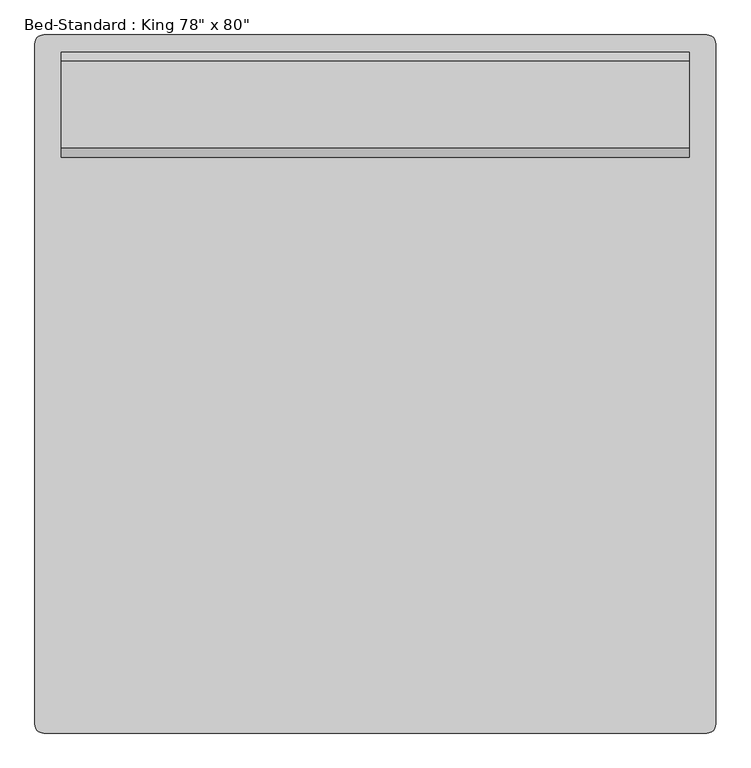
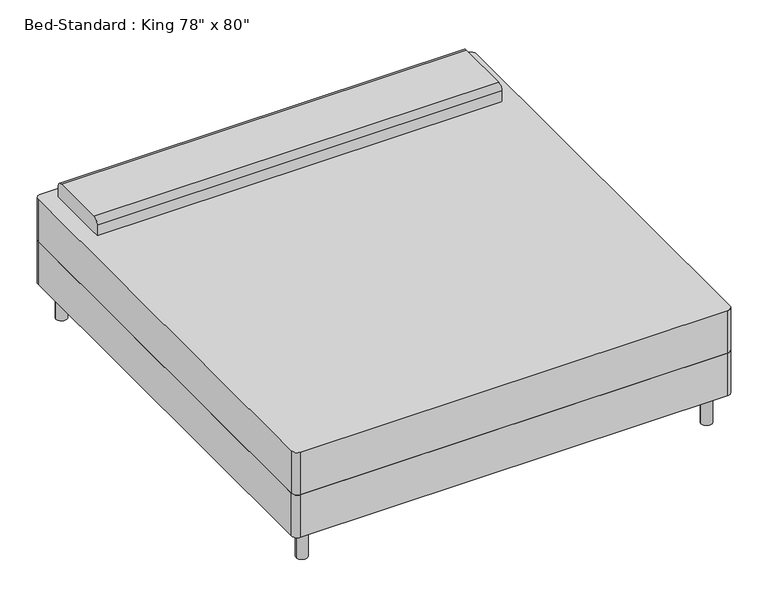
"""IFC4 building model written with IfcOpenShell, lengths in millimetres: furniture geometry."""

import ifcopenshell
import ifcopenshell.guid

model = None  # the IFC model being written
_history = None  # IfcOwnerHistory: only IFC2X3 demands one
_inside = {}  # id of a spatial element -> (the spatial element, [elements in it])
_under = {}  # id of a project, library or spatial element -> (it, [spatial elements below it])
_declared = {}  # id of a project -> (the project, [libraries it declares])
_typed = {}  # id of a type object -> (the type object, [elements of that type])
_made_of = {}  # id of a material, layer set ... -> (it, [elements and type objects made of it])


def new_model(schema):
    """Start an empty IFC model of exactly this schema.

    Asked for "IFC4X3", IfcOpenShell would pick the latest addendum, in which some entities
    have other attributes; the version numbers below select the first issue.
    IFC2X3 requires an IfcOwnerHistory on every rooted entity: one is made here for all.
    """
    global model, _history
    if schema == "IFC4X3":
        model = ifcopenshell.file(schema_version=(4, 3, 0, 0))
    else:
        model = ifcopenshell.file(schema=schema)
    _inside.clear()
    _under.clear()
    _declared.clear()
    _typed.clear()
    _made_of.clear()
    _history = None
    if model.schema == "IFC2X3":
        org = make("IfcOrganization", Name="unknown")
        user = make(
            "IfcPersonAndOrganization",
            ThePerson=make("IfcPerson", FamilyName="unknown"),
            TheOrganization=org,
        )
        app = make(
            "IfcApplication",
            ApplicationDeveloper=org,
            Version="unknown",
            ApplicationFullName="unknown",
            ApplicationIdentifier="unknown",
        )
        _history = make(
            "IfcOwnerHistory",
            OwningUser=user,
            OwningApplication=app,
            ChangeAction="ADDED",
            CreationDate=0,
        )
    return model


def make(cls, **values):
    """One entity of the class cls with the attributes given. An attribute that is None is left unset."""
    return model.create_entity(
        cls, **{name: value for name, value in values.items() if value is not None}
    )


def rooted(cls, **values):
    """An entity with a GlobalId (a new one), such as an element, a storey or a relation."""
    return make(cls, GlobalId=ifcopenshell.guid.new(), OwnerHistory=_history, **values)


def si_unit(unit_type, name, prefix=None):
    """IfcSIUnit, for example si_unit("LENGTHUNIT", "METRE", prefix="MILLI")."""
    return make("IfcSIUnit", UnitType=unit_type, Prefix=prefix, Name=name)


def assignment(units):
    """IfcUnitAssignment: the units of a project."""
    return None if units is None else make("IfcUnitAssignment", Units=units)


def point(xyz):
    """IfcCartesianPoint."""
    return None if xyz is None else make("IfcCartesianPoint", Coordinates=xyz)


def direction(xyz):
    """IfcDirection."""
    return None if xyz is None else make("IfcDirection", DirectionRatios=xyz)


def frame(location, z_axis=None, x_axis=None):
    """IfcAxis2Placement3D, a coordinate frame: its origin and axes. An axis left out is left unset."""
    return make(
        "IfcAxis2Placement3D",
        Location=point(location),
        Axis=direction(z_axis),
        RefDirection=direction(x_axis),
    )


def frame_2d(location, x_axis=None):
    """IfcAxis2Placement2D, a coordinate frame in the plane: its origin and x axis."""
    return make(
        "IfcAxis2Placement2D", Location=point(location), RefDirection=direction(x_axis)
    )


def origin():
    """The frame at (0, 0, 0) with its axes left unset."""
    return frame((0.0, 0.0, 0.0))


def origin_with_axes():
    """The frame at (0, 0, 0) with the z axis (0, 0, 1) and the x axis (1, 0, 0) written out."""
    return frame((0.0, 0.0, 0.0), z_axis=(0.0, 0.0, 1.0), x_axis=(1.0, 0.0, 0.0))


def place(relative_to, where):
    """IfcLocalPlacement: puts the frame where relative to a parent placement (None: the world)."""
    return make(
        "IfcLocalPlacement", PlacementRelTo=relative_to, RelativePlacement=where
    )


def context(
    kind, dimensions, precision=None, world=None, true_north=None, identifier=None
):
    """IfcGeometricRepresentationContext, for example the 3D "Model" context."""
    return make(
        "IfcGeometricRepresentationContext",
        ContextIdentifier=identifier,
        ContextType=kind,
        CoordinateSpaceDimension=dimensions,
        Precision=precision,
        WorldCoordinateSystem=world,
        TrueNorth=true_north,
    )


def project(units=None, contexts=None):
    """IfcProject with its units and contexts."""
    return rooted(
        "IfcProject",
        Name="project",
        RepresentationContexts=contexts,
        UnitsInContext=assignment(units),
    )


def spatial(cls, under=None, at=None, **own):
    """A site, building, storey or space (cls), placed at a placement, below another one or the project."""
    s = rooted(cls, ObjectPlacement=at, **own)
    if under is not None:
        _under.setdefault(under.id(), (under, []))[1].append(s)
    return s


def polyline(points):
    """IfcPolyline through the points."""
    return make("IfcPolyline", Points=[point(p) for p in points])


def circle_curve(where, radius):
    """IfcCircle in the frame where."""
    return make("IfcCircle", Position=where, Radius=radius)


def trimmed(basis, trim1, trim2, sense, master):
    """IfcTrimmedCurve: the piece of a basis curve between two trims."""
    return make(
        "IfcTrimmedCurve",
        BasisCurve=basis,
        Trim1=trim1,
        Trim2=trim2,
        SenseAgreement=sense,
        MasterRepresentation=master,
    )


def segment(curve, same_sense, transition):
    """IfcCompositeCurveSegment."""
    return make(
        "IfcCompositeCurveSegment",
        Transition=transition,
        SameSense=same_sense,
        ParentCurve=curve,
    )


def composite_curve(segments, self_intersect=None):
    """IfcCompositeCurve: segments joined end to end."""
    return make("IfcCompositeCurve", Segments=segments, SelfIntersect=self_intersect)


def outline(outer, holes=None, kind="AREA"):
    """IfcArbitraryClosedProfileDef: a profile drawn as a closed curve; with holes, ...WithVoids."""
    if holes is None:
        return make("IfcArbitraryClosedProfileDef", ProfileType=kind, OuterCurve=outer)
    return make(
        "IfcArbitraryProfileDefWithVoids",
        ProfileType=kind,
        OuterCurve=outer,
        InnerCurves=holes,
    )


def extrude(swept, where, along, depth):
    """IfcExtrudedAreaSolid: the profile swept, set in the frame where, extruded along a direction by depth."""
    return make(
        "IfcExtrudedAreaSolid",
        SweptArea=swept,
        Position=where,
        ExtrudedDirection=direction(along),
        Depth=depth,
    )


def shape(context_of_items, identifier, shape_type, items):
    """IfcShapeRepresentation: the items that make up one representation, for example the "Body"."""
    return make(
        "IfcShapeRepresentation",
        ContextOfItems=context_of_items,
        RepresentationIdentifier=identifier,
        RepresentationType=shape_type,
        Items=items,
    )


def source(mapping_origin, context_of_items, identifier, shape_type, items):
    """IfcRepresentationMap: a shape defined once, which mapped items show again and again."""
    return make(
        "IfcRepresentationMap",
        MappingOrigin=mapping_origin,
        MappedRepresentation=shape(context_of_items, identifier, shape_type, items),
    )


def transform(
    local_origin,
    x_axis=None,
    y_axis=None,
    z_axis=None,
    scale=None,
    scale2=None,
    scale3=None,
    uniform=True,
):
    """IfcCartesianTransformationOperator3D, or its non-uniform kind. x_axis, y_axis, z_axis: its Axis1, 2, 3."""
    if uniform:
        return make(
            "IfcCartesianTransformationOperator3D",
            Axis1=direction(x_axis),
            Axis2=direction(y_axis),
            LocalOrigin=point(local_origin),
            Scale=scale,
            Axis3=direction(z_axis),
        )
    return make(
        "IfcCartesianTransformationOperator3DnonUniform",
        Axis1=direction(x_axis),
        Axis2=direction(y_axis),
        LocalOrigin=point(local_origin),
        Scale=scale,
        Axis3=direction(z_axis),
        Scale2=scale2,
        Scale3=scale3,
    )


def mapped(mapping_source, mapping_target):
    """IfcMappedItem: shows the shape of a source again, moved by a transform."""
    return make(
        "IfcMappedItem", MappingSource=mapping_source, MappingTarget=mapping_target
    )


def made_of(thing, what):
    """Note that an element or type object is made of a material, layer set ...; save() writes the relation."""
    if what is not None:
        _made_of.setdefault(what.id(), (what, []))[1].append(thing)
    return thing


def element(
    cls,
    number,
    at=None,
    inside=None,
    cuts=None,
    type_object=None,
    material=None,
    context=None,
    identifier="Body",
    shape_type=None,
    held_by="IfcProductDefinitionShape",
    body=None,
    shapes=None,
    **own,
):
    """One element of the class cls, such as IfcWall. Its Tag is "e" and its number.

    at: its placement. inside: the storey or other place that contains it. cuts: it is an
    opening in that element (IfcRelVoidsElement). A single representation is given by context,
    identifier, shape_type and body (its items); several are given by shapes. held_by: the class
    of the entity that holds the representations. save() writes the other relations.
    """
    e = rooted(cls, Tag="e%d" % number, ObjectPlacement=at, **own)
    if body is not None:
        shapes = [shape(context, identifier, shape_type, body)]
    if shapes is not None:
        e.Representation = make(held_by, Representations=shapes)
    if inside is not None:
        _inside.setdefault(inside.id(), (inside, []))[1].append(e)
    if cuts is not None:
        rooted(
            "IfcRelVoidsElement", RelatingBuildingElement=cuts, RelatedOpeningElement=e
        )
    if type_object is not None:
        _typed.setdefault(type_object.id(), (type_object, []))[1].append(e)
    return made_of(e, material)


def aggregate(whole, parts):
    """IfcRelAggregates: a whole, such as a stair, and the parts it consists of."""
    return rooted("IfcRelAggregates", RelatingObject=whole, RelatedObjects=parts)


def save(model, path):
    """Write the relations noted so far, then the file.

    IfcRelAggregates (storeys below a building ...), IfcRelContainedInSpatialStructure (elements
    in a storey), IfcRelDefinesByType, IfcRelAssociatesMaterial and IfcRelDeclares: one each for
    every whole, place, type object, material and project.
    """
    for whole, parts in _under.values():
        aggregate(whole, parts)
    for where, things in _inside.values():
        rooted(
            "IfcRelContainedInSpatialStructure",
            RelatedElements=things,
            RelatingStructure=where,
        )
    for kind, things in _typed.values():
        rooted("IfcRelDefinesByType", RelatedObjects=things, RelatingType=kind)
    for what, things in _made_of.values():
        rooted("IfcRelAssociatesMaterial", RelatedObjects=things, RelatingMaterial=what)
    for by, libraries in _declared.values():
        rooted("IfcRelDeclares", RelatingContext=by, RelatedDefinitions=libraries)
    model.write(path)


def furniture_1fc5af50(model_context):
    return source(origin(), model_context, "Body", "SweptSolid", [
        extrude(outline(composite_curve([segment(polyline([(-719.1114754, -1036.195082), (-719.1114754, 945.004918)]), True, "CONTINUOUS"), segment(trimmed(circle_curve(frame_2d((-693.7114754, 945.004918)), 25.4), [point((-719.1114754, 945.004918))], [point((-693.7114754, 970.404918))], False, "CARTESIAN"), True, "CONTINUOUS"), segment(polyline([(-693.7114754, 970.404918), (1236.6885246, 970.404918)]), True, "CONTINUOUS"), segment(trimmed(circle_curve(frame_2d((1236.6885246, 945.004918)), 25.4), [point((1236.6885246, 970.404918))], [point((1262.0885246, 945.004918))], False, "CARTESIAN"), True, "CONTINUOUS"), segment(polyline([(1262.0885246, 945.004918), (1262.0885246, -1036.195082)]), True, "CONTINUOUS"), segment(trimmed(circle_curve(frame_2d((1236.6885246, -1036.195082)), 25.4), [point((1262.0885246, -1036.195082))], [point((1236.6885246, -1061.595082))], False, "CARTESIAN"), True, "CONTINUOUS"), segment(polyline([(1236.6885246, -1061.595082), (-693.7114754, -1061.595082)]), True, "CONTINUOUS"), segment(trimmed(circle_curve(frame_2d((-693.7114754, -1036.195082)), 25.4), [point((-693.7114754, -1061.595082))], [point((-719.1114754, -1036.195082))], False, "CARTESIAN"), True, "CONTINUOUS")], self_intersect=False)), frame((0.0, 0.0, 152.4), z_axis=(0.0, 0.0, 1.0), x_axis=(1.0, 0.0, 0.0)), (0.0, 0.0, 1.0), 203.2),
        extrude(outline(composite_curve([segment(polyline([(614.804918, 558.8), (614.804918, 609.6)]), True, "CONTINUOUS"), segment(trimmed(circle_curve(frame_2d((640.204918, 609.6)), 25.4), [point((614.804918, 609.6))], [point((640.204918, 635.0))], False, "CARTESIAN"), True, "CONTINUOUS"), segment(polyline([(640.204918, 635.0), (894.204918, 635.0)]), True, "CONTINUOUS"), segment(trimmed(circle_curve(frame_2d((894.204918, 609.6)), 25.4), [point((894.204918, 635.0))], [point((919.604918, 609.6))], False, "CARTESIAN"), True, "CONTINUOUS"), segment(polyline([(919.604918, 609.6), (919.604918, 558.8), (614.804918, 558.8)]), True, "CONTINUOUS")], self_intersect=False)), frame((-642.9114754, 0.0, 0.0), z_axis=(1.0, 0.0, 0.0), x_axis=(0.0, 1.0, 0.0)), (0.0, 0.0, 1.0), 1828.8),
        extrude(outline(composite_curve([segment(trimmed(circle_curve(frame_2d((-642.9114754, 894.204918)), 25.4), [point((-668.3114754, 894.204918))], [point((-617.5114754, 894.204918))], False, "CARTESIAN"), True, "CONTINUOUS"), segment(trimmed(circle_curve(frame_2d((-642.9114754, 894.204918)), 25.4), [point((-617.5114754, 894.204918))], [point((-668.3114754, 894.204918))], False, "CARTESIAN"), True, "CONTINUOUS")], self_intersect=False)), origin_with_axes(), (0.0, 0.0, 1.0), 152.4),
        extrude(outline(composite_curve([segment(trimmed(circle_curve(frame_2d((1185.8885246, 894.204918)), 25.4), [point((1160.4885246, 894.204918))], [point((1211.2885246, 894.204918))], False, "CARTESIAN"), True, "CONTINUOUS"), segment(trimmed(circle_curve(frame_2d((1185.8885246, 894.204918)), 25.4), [point((1211.2885246, 894.204918))], [point((1160.4885246, 894.204918))], False, "CARTESIAN"), True, "CONTINUOUS")], self_intersect=False)), origin_with_axes(), (0.0, 0.0, 1.0), 152.4),
        extrude(outline(composite_curve([segment(trimmed(circle_curve(frame_2d((1185.8885246, -985.395082)), 25.4), [point((1160.4885246, -985.395082))], [point((1211.2885246, -985.395082))], False, "CARTESIAN"), True, "CONTINUOUS"), segment(trimmed(circle_curve(frame_2d((1185.8885246, -985.395082)), 25.4), [point((1211.2885246, -985.395082))], [point((1160.4885246, -985.395082))], False, "CARTESIAN"), True, "CONTINUOUS")], self_intersect=False)), origin_with_axes(), (0.0, 0.0, 1.0), 152.4),
        extrude(outline(composite_curve([segment(trimmed(circle_curve(frame_2d((-642.9114754, -985.395082)), 25.4), [point((-668.3114754, -985.395082))], [point((-617.5114754, -985.395082))], False, "CARTESIAN"), True, "CONTINUOUS"), segment(trimmed(circle_curve(frame_2d((-642.9114754, -985.395082)), 25.4), [point((-617.5114754, -985.395082))], [point((-668.3114754, -985.395082))], False, "CARTESIAN"), True, "CONTINUOUS")], self_intersect=False)), origin_with_axes(), (0.0, 0.0, 1.0), 152.4),
        extrude(outline(composite_curve([segment(polyline([(-693.7114754, 970.404918), (1236.6885246, 970.404918)]), True, "CONTINUOUS"), segment(trimmed(circle_curve(frame_2d((1236.6885246, 945.004918)), 25.4), [point((1236.6885246, 970.404918))], [point((1262.0885246, 945.004918))], False, "CARTESIAN"), True, "CONTINUOUS"), segment(polyline([(1262.0885246, 945.004918), (1262.0885246, -1036.195082)]), True, "CONTINUOUS"), segment(trimmed(circle_curve(frame_2d((1236.6885246, -1036.195082)), 25.4), [point((1262.0885246, -1036.195082))], [point((1236.6885246, -1061.595082))], False, "CARTESIAN"), True, "CONTINUOUS"), segment(polyline([(1236.6885246, -1061.595082), (-693.7114754, -1061.595082)]), True, "CONTINUOUS"), segment(trimmed(circle_curve(frame_2d((-693.7114754, -1036.195082)), 25.4), [point((-693.7114754, -1061.595082))], [point((-719.1114754, -1036.195082))], False, "CARTESIAN"), True, "CONTINUOUS"), segment(polyline([(-719.1114754, -1036.195082), (-719.1114754, 945.004918)]), True, "CONTINUOUS"), segment(trimmed(circle_curve(frame_2d((-693.7114754, 945.004918)), 25.4), [point((-719.1114754, 945.004918))], [point((-693.7114754, 970.404918))], False, "CARTESIAN"), True, "CONTINUOUS")], self_intersect=False)), frame((0.0, 0.0, 355.6), z_axis=(0.0, 0.0, 1.0), x_axis=(1.0, 0.0, 0.0)), (0.0, 0.0, 1.0), 203.2),
    ])


if __name__ == "__main__":
    model = new_model("IFC4")
    model_context = context("Model", 3, world=origin())
    ifc_project = project(units=[si_unit("LENGTHUNIT", "METRE", prefix="MILLI")], contexts=[model_context])
    site = spatial("IfcSite", under=ifc_project)
    building = spatial("IfcBuilding", under=site)
    placement = place(None, origin())
    furniture_shape = furniture_1fc5af50(model_context)
    element("IfcFurniture", 1, ObjectType="Bed-Standard : King 78\" x 80\"", at=placement, inside=building, context=model_context, shape_type="MappedRepresentation", body=[
        mapped(furniture_shape, transform((0.0, 0.0, 0.0), x_axis=(1.0, 0.0, 0.0), y_axis=(0.0, 1.0, 0.0), z_axis=(0.0, 0.0, 1.0))),
    ])
    save(model, "model.ifc")

# Revit data of these elements
# Type "Bed-Standard : King 78\" x 80\""
#   Model = "King Bed"
#   Manufacturer = "Acme Funriture"
#   Assembly Code = "E2020200"
#   Length = 6' - 8"
#   Width = 6' - 6"
#   Leg Material = Metal - Chrome
#   Mattress Material = Textile - White
#   Type Comments = ""
#   Default Elevation = 0
# Element 1 (IfcFurniture, "Bed-Standard : King 78\" x 80\"")
#   Materials on its faces: "Textile - White", "Metal - Chrome"
# Materials
#   "Metal - Chrome": class "Unassigned", colour RGB 17 17 17, transparency 0, Description = "Chrome"
#   "Textile - White": class "Unassigned", colour RGB 247 247 239, transparency 0
